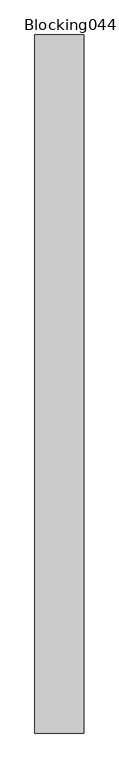
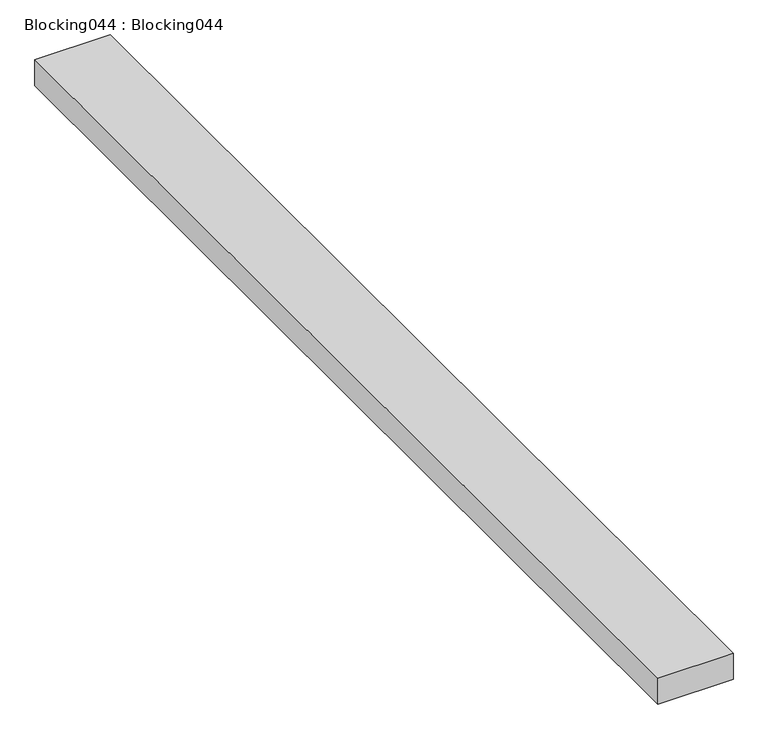
"""IFC4 building model written with IfcOpenShell, lengths in millimetres: proxy geometry, Blocking044 : Blocking044."""

from ifc_helpers import new_model, si_unit, frame, origin, place, context, project, spatial, polyline, outline, extrude, source, transform, mapped, element, save


def blocking044_blocking044_f67fe0f3(model_context):
    return source(origin(), model_context, "Body", "SweptSolid", [
        extrude(outline(polyline([(-950.3815411, -1052.8908936), (-1090.0815411, -1052.8908936), (-1090.0815411, 947.1091064), (-950.3815411, 947.1091064), (-950.3815411, -1052.8908936)])), frame((0.0, 0.0, 40112.696), z_axis=(0.0, 0.0, 1.0), x_axis=(1.0, 0.0, 0.0)), (0.0, 0.0, 1.0), 50.8),
    ])


if __name__ == "__main__":
    model = new_model("IFC4")
    model_context = context("Model", 3, world=origin())
    ifc_project = project(units=[si_unit("LENGTHUNIT", "METRE", prefix="MILLI")], contexts=[model_context])
    site = spatial("IfcSite", under=ifc_project)
    building = spatial("IfcBuilding", under=site)
    placement = place(None, origin())
    blocking044_blocking044_shape = blocking044_blocking044_f67fe0f3(model_context)
    element("IfcBuildingElementProxy", 1, Name="Blocking044 : Blocking044", ObjectType="Blocking044 : Blocking044", at=placement, inside=building, context=model_context, shape_type="MappedRepresentation", body=[
        mapped(blocking044_blocking044_shape, transform((0.0, 0.0, 0.0), x_axis=(1.0, 0.0, 0.0), y_axis=(0.0, 1.0, 0.0), z_axis=(0.0, 0.0, 1.0))),
    ])
    save(model, "model.ifc")

# Revit data of these elements
# Type "Blocking044 : Blocking044"
#   NameOverride = "Blocking044"
# Element 1 (IfcBuildingElementProxy, "Blocking044 : Blocking044")
#   Materials on its faces: "WOOD BLOCKING AS REQUIRED"
# Materials
#   "WOOD BLOCKING AS REQUIRED": class "Unassigned", colour RGB 166 124 85, transparency 0, Cost = 0
